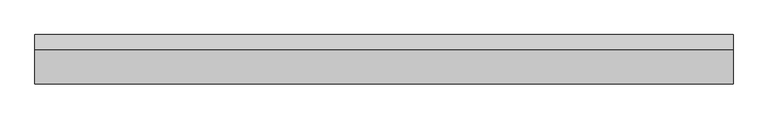
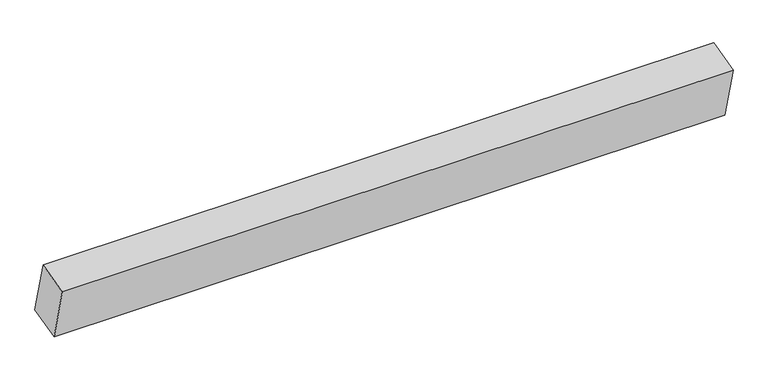
"""IFC4 building model written with IfcOpenShell, lengths in millimetres: proxy geometry, Insulation012 1108 : Insulation012 1108."""

from ifc_helpers import new_model, si_unit, frame, origin, place, context, project, spatial, polyline, outline, extrude, source, transform, mapped, element, save


def generic_models_79768f30(model_context):
    return source(origin(), model_context, "Body", "SweptSolid", [
        extrude(outline(polyline([(10280.4083448, 43740.2868413), (10322.2187966, 43573.045034), (10222.2072294, 43548.0351751), (10180.3882058, 43715.2646709), (10280.4083448, 43740.2868413)])), frame((3694.2883192, 0.0, 0.0), z_axis=(1.0, 0.0, 0.0), x_axis=(0.0, 1.0, 0.0)), (0.0, 0.0, 1.0), 2000.0),
    ])


if __name__ == "__main__":
    model = new_model("IFC4")
    model_context = context("Model", 3, world=origin())
    ifc_project = project(units=[si_unit("LENGTHUNIT", "METRE", prefix="MILLI")], contexts=[model_context])
    site = spatial("IfcSite", under=ifc_project)
    building = spatial("IfcBuilding", under=site)
    placement = place(None, origin())
    generic_models_shape = generic_models_79768f30(model_context)
    element("IfcBuildingElementProxy", 1, Name="Insulation012 1108 : Insulation012 1108", ObjectType="Insulation012 1108 : Insulation012 1108", at=placement, inside=building, context=model_context, shape_type="MappedRepresentation", body=[
        mapped(generic_models_shape, transform((0.0, 0.0, 0.0), x_axis=(1.0, 0.0, 0.0), y_axis=(0.0, 1.0, 0.0), z_axis=(0.0, 0.0, 1.0))),
    ])
    save(model, "model.ifc")

# Revit data of these elements
# Type "Insulation012 1108 : Insulation012 1108"
#   NameOverride = "Insulation012"
# Element 1 (IfcBuildingElementProxy, "Insulation012 1108 : Insulation012 1108")
#   Materials on its faces: "BATT INSULATION (U-FACTOR = 0.065 MIN.) OVER CLASS II VAPOR RETARDER (TOWARDS INTERIOR)"
# Materials
#   "BATT INSULATION (U-FACTOR = 0.065 MIN.) OVER CLASS II VAPOR RETARDER (TOWARDS INTERIOR)": class "Unassigned", colour RGB 246 242 160, transparency 0, Cost = 0
